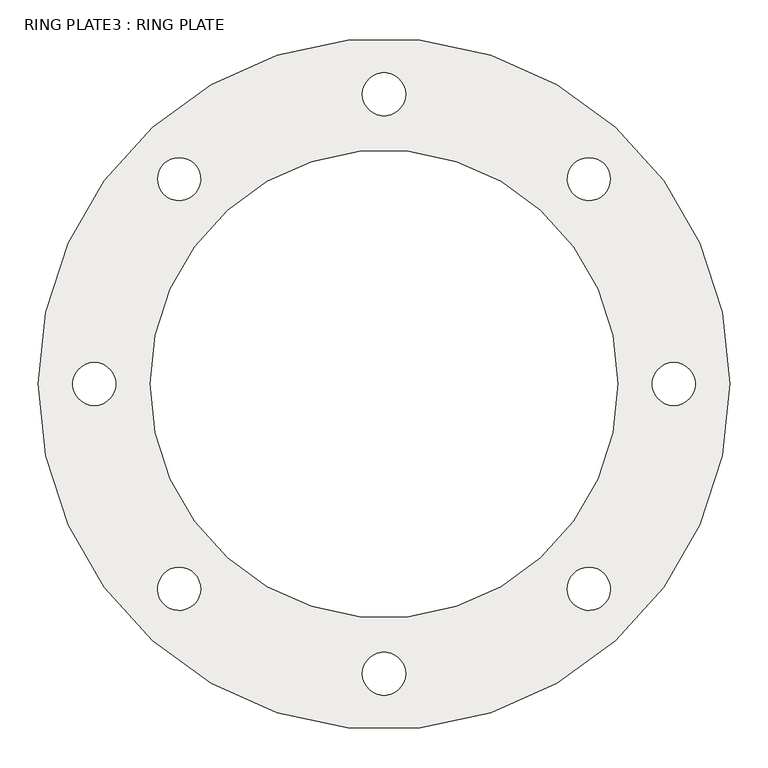
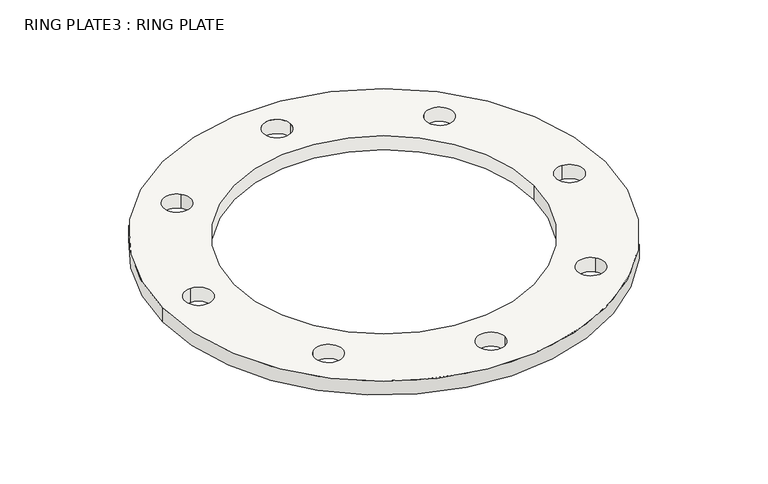
"""IFC4 building model written with IfcOpenShell, lengths in millimetres: slab geometry, RING PLATE3 : RING PLATE."""

from ifc_helpers import new_model, si_unit, point, frame, frame_2d, origin, place, context, project, spatial, circle_curve, trimmed, segment, composite_curve, outline, extrude, source, transform, mapped, element, save


def ring_plate3_ring_plate_67d48941(model_context):
    return source(origin(), model_context, "Body", "SweptSolid", [
        extrude(outline(composite_curve([segment(trimmed(circle_curve(frame_2d((-30945.7763606, -7583.9705533)), 450.0), [point((-31395.7763606, -7583.9705533))], [point((-30495.7763606, -7583.9705533))], False, "CARTESIAN"), True, "CONTINUOUS"), segment(trimmed(circle_curve(frame_2d((-30945.7763606, -7583.9705533)), 450.0), [point((-30495.7763606, -7583.9705533))], [point((-31395.7763606, -7583.9705533))], False, "CARTESIAN"), True, "CONTINUOUS")], self_intersect=False), holes=[composite_curve([segment(trimmed(circle_curve(frame_2d((-30945.7763606, -7583.9705533)), 304.5), [point((-31250.2763606, -7583.9705533))], [point((-30641.2763606, -7583.9705533))], True, "CARTESIAN"), True, "CONTINUOUS"), segment(trimmed(circle_curve(frame_2d((-30945.7763606, -7583.9705533)), 304.5), [point((-30641.2763606, -7583.9705533))], [point((-31250.2763606, -7583.9705533))], True, "CARTESIAN"), True, "CONTINUOUS")], self_intersect=False), composite_curve([segment(trimmed(circle_curve(frame_2d((-30945.7763606, -7961.2205533)), 28.0044639), [point((-30973.7808246, -7961.2205533))], [point((-30917.7718967, -7961.2205533))], True, "CARTESIAN"), True, "CONTINUOUS"), segment(trimmed(circle_curve(frame_2d((-30945.7763606, -7961.2205533)), 28.0044639), [point((-30917.7718967, -7961.2205533))], [point((-30973.7808246, -7961.2205533))], True, "CARTESIAN"), True, "CONTINUOUS")], self_intersect=False), composite_curve([segment(trimmed(circle_curve(frame_2d((-31212.5323938, -7850.7265865)), 28.0), [point((-31232.3313837, -7830.9275967))], [point((-31192.733404, -7870.5255764))], True, "CARTESIAN"), True, "CONTINUOUS"), segment(trimmed(circle_curve(frame_2d((-31212.5323938, -7850.7265865)), 28.0), [point((-31192.733404, -7870.5255764))], [point((-31232.3313837, -7830.9275967))], True, "CARTESIAN"), True, "CONTINUOUS")], self_intersect=False), composite_curve([segment(trimmed(circle_curve(frame_2d((-31323.0263606, -7583.9705533)), 28.0), [point((-31323.0263606, -7555.9705533))], [point((-31323.0263606, -7611.9705533))], True, "CARTESIAN"), True, "CONTINUOUS"), segment(trimmed(circle_curve(frame_2d((-31323.0263606, -7583.9705533)), 28.0), [point((-31323.0263606, -7611.9705533))], [point((-31323.0263606, -7555.9705533))], True, "CARTESIAN"), True, "CONTINUOUS")], self_intersect=False), composite_curve([segment(trimmed(circle_curve(frame_2d((-31212.5323938, -7317.2145201)), 28.0), [point((-31192.733404, -7297.4155303))], [point((-31232.3313837, -7337.01351))], True, "CARTESIAN"), True, "CONTINUOUS"), segment(trimmed(circle_curve(frame_2d((-31212.5323938, -7317.2145201)), 28.0), [point((-31232.3313837, -7337.01351))], [point((-31192.733404, -7297.4155303))], True, "CARTESIAN"), True, "CONTINUOUS")], self_intersect=False), composite_curve([segment(trimmed(circle_curve(frame_2d((-30945.7763606, -7206.7205533)), 28.0), [point((-30917.7763606, -7206.7205533))], [point((-30973.7763606, -7206.7205533))], True, "CARTESIAN"), True, "CONTINUOUS"), segment(trimmed(circle_curve(frame_2d((-30945.7763606, -7206.7205533)), 28.0), [point((-30973.7763606, -7206.7205533))], [point((-30917.7763606, -7206.7205533))], True, "CARTESIAN"), True, "CONTINUOUS")], self_intersect=False), composite_curve([segment(trimmed(circle_curve(frame_2d((-30679.0203274, -7317.2145201)), 28.0), [point((-30659.2213376, -7337.01351))], [point((-30698.8193173, -7297.4155303))], True, "CARTESIAN"), True, "CONTINUOUS"), segment(trimmed(circle_curve(frame_2d((-30679.0203274, -7317.2145201)), 28.0), [point((-30698.8193173, -7297.4155303))], [point((-30659.2213376, -7337.01351))], True, "CARTESIAN"), True, "CONTINUOUS")], self_intersect=False), composite_curve([segment(trimmed(circle_curve(frame_2d((-30568.5263606, -7583.9705533)), 28.0), [point((-30568.5263606, -7611.9705533))], [point((-30568.5263606, -7555.9705533))], True, "CARTESIAN"), True, "CONTINUOUS"), segment(trimmed(circle_curve(frame_2d((-30568.5263606, -7583.9705533)), 28.0), [point((-30568.5263606, -7555.9705533))], [point((-30568.5263606, -7611.9705533))], True, "CARTESIAN"), True, "CONTINUOUS")], self_intersect=False), composite_curve([segment(trimmed(circle_curve(frame_2d((-30679.0203274, -7850.7265865)), 28.0), [point((-30698.8193173, -7870.5255764))], [point((-30659.2213376, -7830.9275967))], True, "CARTESIAN"), True, "CONTINUOUS"), segment(trimmed(circle_curve(frame_2d((-30679.0203274, -7850.7265865)), 28.0), [point((-30659.2213376, -7830.9275967))], [point((-30698.8193173, -7870.5255764))], True, "CARTESIAN"), True, "CONTINUOUS")], self_intersect=False)]), frame((0.0, 0.0, 130.0), z_axis=(0.0, 0.0, 1.0), x_axis=(1.0, 0.0, 0.0)), (0.0, 0.0, 1.0), 30.0),
    ])


if __name__ == "__main__":
    model = new_model("IFC4")
    model_context = context("Model", 3, world=origin())
    ifc_project = project(units=[si_unit("LENGTHUNIT", "METRE", prefix="MILLI")], contexts=[model_context])
    site = spatial("IfcSite", under=ifc_project)
    building = spatial("IfcBuilding", under=site)
    placement = place(None, origin())
    ring_plate3_ring_plate_shape = ring_plate3_ring_plate_67d48941(model_context)
    element("IfcSlab", 1, ObjectType="RING PLATE3 : RING PLATE", at=placement, inside=building, context=model_context, shape_type="MappedRepresentation", body=[
        mapped(ring_plate3_ring_plate_shape, transform((0.0, 0.0, 0.0), x_axis=(1.0, 0.0, 0.0), y_axis=(0.0, 1.0, 0.0), z_axis=(0.0, 0.0, 1.0))),
    ])
    save(model, "model.ifc")
